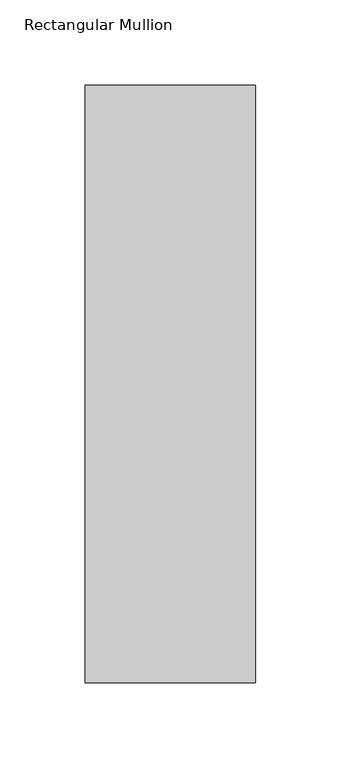
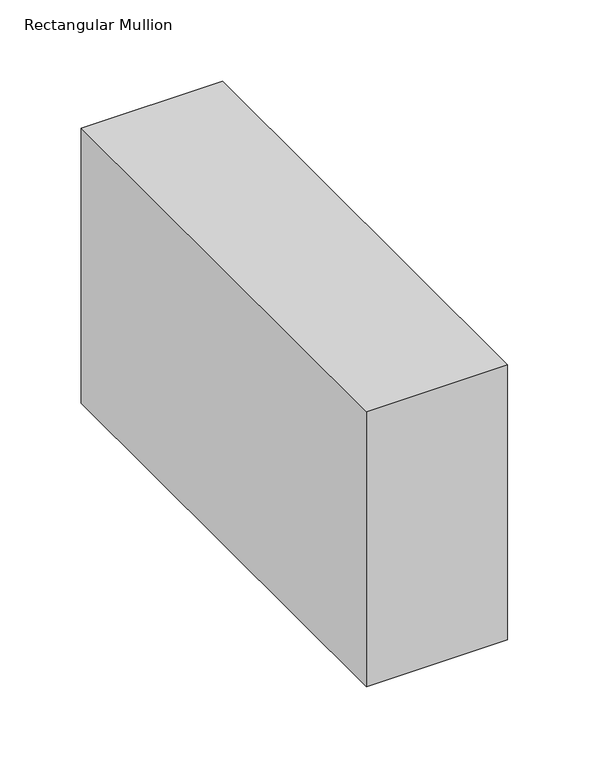
"""IFC4 building model written with IfcOpenShell, lengths in millimetres: member geometry, Rectangular Mullion : WWm-100x350-100mmOffset."""

from ifc_helpers import new_model, si_unit, frame, origin, place, context, project, spatial, polyline, outline, extrude, source, transform, mapped, element, save


def rectangular_mullion_37c9cdfb(model_context):
    return source(origin(), model_context, "Body", "SweptSolid", [
        extrude(outline(polyline([(0.0, 175.0), (0.0, -175.0), (-100.0, -175.0), (-100.0, 175.0), (0.0, 175.0)])), frame((0.0, 0.0, -205.9981454), z_axis=(0.0, 0.0, 1.0), x_axis=(1.0, 0.0, 0.0)), (0.0, 0.0, 1.0), 205.9981454),
    ])


if __name__ == "__main__":
    model = new_model("IFC4")
    model_context = context("Model", 3, world=origin())
    ifc_project = project(units=[si_unit("LENGTHUNIT", "METRE", prefix="MILLI")], contexts=[model_context])
    site = spatial("IfcSite", under=ifc_project)
    building = spatial("IfcBuilding", under=site)
    placement = place(None, origin())
    rectangular_mullion_shape = rectangular_mullion_37c9cdfb(model_context)
    element("IfcMember", 1, ObjectType="Rectangular Mullion : WWm-100x350-100mmOffset", at=placement, inside=building, context=model_context, shape_type="MappedRepresentation", body=[
        mapped(rectangular_mullion_shape, transform((0.0, 0.0, 0.0), x_axis=(1.0, 0.0, 0.0), y_axis=(0.0, 1.0, 0.0), z_axis=(0.0, 0.0, 1.0))),
    ])
    save(model, "model.ifc")

# Revit data of these elements
# Type "Rectangular Mullion : WWm-100x350-100mmOffset"
#   built-in parameter 1007304 = 1.14829 (stored number, unit not read)
#   built-in parameter 1007301 = 0.164042 (stored number, unit not read)
#   built-in parameter 1007300 = 0.164042 (stored number, unit not read)
# Element 1 (IfcMember, "Rectangular Mullion : WWm-100x350-100mmOffset")
#   Materials on its faces: "WW-EC-RGB-Mullion"
# Materials
#   "WW-EC-RGB-Mullion": class "Generic", colour RGB 255 255 255, transparency 0, Comments = "If region requests black mullions, switch asset color to RGB 25-25-25", Description = "Generic Color", Cost = 0
